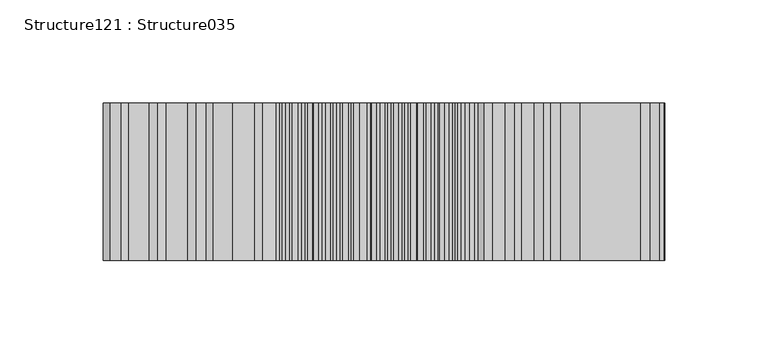
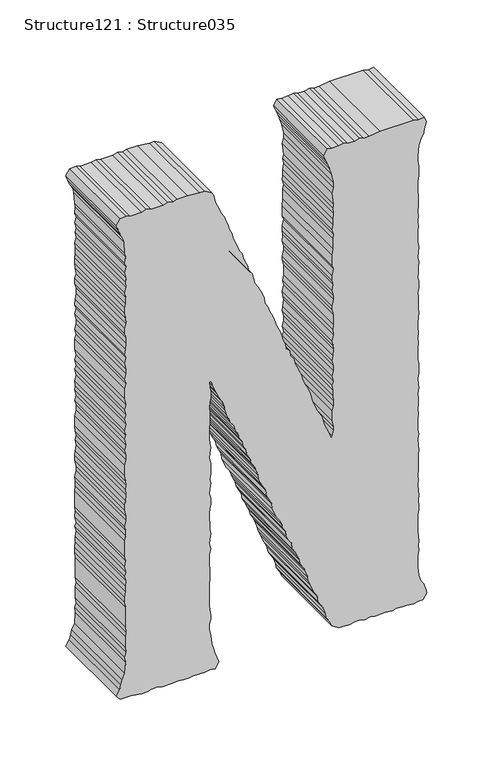
"""IFC4 building model written with IfcOpenShell, lengths in millimetres: proxy geometry, Structure121 : Structure035."""

from ifc_helpers import new_model, si_unit, frame, origin, place, context, project, spatial, polyline, outline, extrude, source, transform, mapped, element, save


def structure121_structure035_140282e5(model_context):
    return source(origin(), model_context, "Body", "SweptSolid", [
        extrude(outline(polyline([(3575.0851816, -43990.4752466), (3583.2863152, -43991.6353756), (3589.1527492, -43992.8163645), (3593.8285667, -43992.8163645), (3597.9540049, -43991.6353756), (3602.0280957, -43991.6353756), (3607.3393366, -43992.2371023), (3611.4134274, -43992.8163645), (3631.3410106, -43992.8163645), (3635.4407751, -43992.2371023), (3644.8245022, -43992.2371023), (3648.9258713, -43992.8163645), (3658.3015753, -43992.8163645), (3663.5598643, -43991.6353756), (3668.2437048, -43992.8163645), (3672.3691429, -43992.2371023), (3677.0449604, -43991.6353756), (3681.7271964, -43992.2371023), (3687.587212, -43992.2371023), (3691.6869765, -43992.8163645), (3696.3884676, -43992.8163645), (3700.4705815, -43992.2371023), (3704.5879966, -43991.6353756), (3709.8559132, -43991.6353756), (3714.5301261, -43992.8163645), (3718.6571688, -43992.2371023), (3723.9154578, -43991.6353756), (3728.0152223, -43992.2371023), (3732.7167134, -43991.6353756), (3742.6748889, -43991.6353756), (3747.3587295, -43992.8163645), (3752.6170184, -43992.2371023), (3757.3185096, -43991.6353756), (3760.818152, -43992.2371023), (3766.684586, -43992.8163645), (3774.8857196, -43992.8163645), (3780.7441306, -43992.2371023), (3790.1294623, -43992.2371023), (3794.2292268, -43992.8163645), (3798.9050443, -43992.2371023), (3803.0064134, -43991.6353756), (3808.8888934, -43991.6353756), (3812.9726119, -43992.2371023), (3818.2309008, -43992.8163645), (3817.6741031, -43991.6353756), (3812.9726119, -43989.2942576), (3808.290376, -43987.5340065), (3804.7730829, -43985.7962198), (3800.6717138, -43984.6152309), (3795.960595, -43981.6948508), (3790.7039107, -43979.9121352), (3787.2042683, -43978.7536107), (3782.5027771, -43977.5726218), (3777.8285642, -43975.8123707), (3773.7015215, -43974.0729794), (3770.2018791, -43971.1317394), (3766.1021146, -43969.9732149), (3760.2437036, -43967.632097), (3757.3185096, -43966.451108), (3752.6170184, -43964.1115947), (3748.5429276, -43962.9306058), (3743.8414364, -43960.5894878), (3739.1592005, -43960.0102256), (3733.8736333, -43957.09145), (3730.3563402, -43955.9104611), (3725.6741043, -43953.5484833), (3722.1568112, -43951.809092), (3716.8985223, -43950.0488409), (3712.7971532, -43949.4695787), (3708.087639, -43947.7093275), (3703.4134261, -43945.3682096), (3700.4705815, -43943.6079584), (3694.6298211, -43942.4269695), (3691.0868544, -43940.6667184), (3686.4030139, -43938.3256004), (3681.7271964, -43937.7463382), (3672.9435914, -43934.225836), (3668.8261762, -43931.2845959), (3664.1423357, -43929.5452046), (3660.6250426, -43928.3642157), (3655.9428067, -43926.0247024), (3651.8590883, -43925.4454402), (3647.1575971, -43923.1043222), (3643.6579547, -43920.7423444), (3638.3563415, -43920.1630822), (3634.2822506, -43917.8235688), (3630.1824862, -43916.0617131), (3625.472972, -43913.7221997), (3621.3732075, -43913.120473), (3616.69739, -43910.2016975), (3613.1720739, -43908.4398417), (3607.3393366, -43906.6795906), (3603.7963698, -43906.1003284), (3599.7126514, -43904.3400772), (3591.5131224, -43900.8179704), (3586.8116312, -43898.478457), (3581.5276686, -43897.2974681), (3577.4535778, -43894.9579547), (3573.3265351, -43892.6168368), (3568.0682461, -43890.8565857), (3563.9412034, -43890.2773234), (3559.2669905, -43887.3585479), (3555.1848766, -43885.5966921), (3551.0658569, -43879.7366765), (3551.0658569, -43875.6353074), (3550.4833855, -43870.3529494), (3551.6675836, -43865.6739227), (3551.6675836, -43862.1518158), (3550.4833855, -43856.8710624), (3551.6675836, -43852.1904311), (3550.4833855, -43848.089062), (3551.0658569, -43842.2290464), (3551.0658569, -43838.729404), (3550.4833855, -43832.8677838), (3551.6675836, -43829.3472815), (3551.0658569, -43824.0649235), (3551.0658569, -43819.965159), (3550.4833855, -43814.1260033), (3551.0658569, -43810.0021697), (3551.0658569, -43805.9024052), (3556.3417965, -43802.4027628), (3559.8671125, -43803.5612873), (3565.7094775, -43805.323143), (3569.2524442, -43807.6626564), (3575.0851816, -43809.4229075), (3583.2863152, -43810.6038964), (3593.2541183, -43810.6038964), (3598.5284533, -43809.4229075), (3602.0280957, -43810.0021697), (3607.3393366, -43809.4229075), (3611.4134274, -43810.0021697), (3616.69739, -43810.6038964), (3631.3410106, -43810.6038964), (3635.4407751, -43809.4229075), (3640.114988, -43809.4229075), (3644.2420307, -43810.0021697), (3650.1004418, -43809.4229075), (3653.6000842, -43810.0021697), (3659.4584952, -43810.6038964), (3662.9854159, -43810.0021697), (3668.2437048, -43810.6038964), (3672.3691429, -43810.0021697), (3687.0127636, -43810.0021697), (3691.0868544, -43809.4229075), (3695.786741, -43810.0021697), (3701.6547796, -43810.6038964), (3705.7545441, -43809.4229075), (3709.8559132, -43810.6038964), (3719.2316172, -43810.6038964), (3725.0996559, -43810.0021697), (3728.5992983, -43810.6038964), (3734.47536, -43810.0021697), (3739.1592005, -43810.0021697), (3743.8414364, -43810.6038964), (3748.5429276, -43809.4229075), (3752.04257, -43810.0021697), (3757.8753073, -43810.6038964), (3762.0023501, -43809.4229075), (3771.3860772, -43809.4229075), (3775.4874463, -43810.6038964), (3784.8438951, -43810.6038964), (3790.1294623, -43810.0021697), (3795.4037973, -43810.6038964), (3799.5051664, -43810.0021697), (3804.7730829, -43810.6038964), (3809.4729695, -43810.6038964), (3812.9726119, -43810.0021697), (3818.2309008, -43809.4229075), (3822.348316, -43810.0021697), (3832.3161191, -43810.0021697), (3836.9919366, -43810.6038964), (3841.0900965, -43809.4229075), (3846.9757858, -43809.4229075), (3850.4754282, -43810.6038964), (3855.7353217, -43810.0021697), (3859.8591552, -43810.0021697), (3865.1190488, -43809.4229075), (3869.8189354, -43810.6038964), (3879.1769888, -43809.4229075), (3883.8881076, -43810.6038964), (3893.246161, -43810.6038964), (3898.5301236, -43810.0021697), (3903.2059411, -43810.6038964), (3907.3313793, -43810.0021697), (3912.0071968, -43810.6038964), (3916.6653636, -43810.0021697), (3926.6492128, -43810.0021697), (3930.1745289, -43810.6038964), (3940.1166583, -43810.6038964), (3944.8165449, -43809.4229075), (3953.5937315, -43809.4229075), (3959.4617701, -43810.6038964), (3962.9774586, -43810.6038964), (3972.9372387, -43809.4229075), (3977.6194746, -43807.6626564), (3982.8793681, -43805.323143), (3986.4046842, -43804.7422762), (3992.2614906, -43802.9820251), (3996.9645864, -43804.7422762), (3996.390138, -43809.4229075), (3997.5486624, -43814.1260033), (3997.5486624, -43843.4100353), (3996.390138, -43852.7696933), (3996.390138, -43857.4727891), (3997.5486624, -43860.9932914), (3996.390138, -43865.6739227), (3996.390138, -43871.5339383), (3997.5486624, -43875.0335807), (3996.9645864, -43879.7366765), (3996.9645864, -43885.5966921), (3997.5486624, -43889.6980612), (3992.2614906, -43892.6168368), (3987.5792547, -43890.8565857), (3982.3225704, -43888.5170723), (3978.2035506, -43887.3585479), (3972.9372387, -43885.5966921), (3964.1343784, -43883.836441), (3959.4617701, -43883.836441), (3954.7506513, -43885.0174299), (3944.235678, -43883.836441), (3940.718385, -43884.4157032), (3936.0345445, -43883.836441), (3930.7329312, -43884.4157032), (3925.4746423, -43884.4157032), (3921.3748778, -43885.0174299), (3916.6653636, -43883.836441), (3912.5896682, -43884.4157032), (3903.2059411, -43884.4157032), (3897.3475301, -43885.0174299), (3887.9621984, -43885.0174299), (3884.4609514, -43883.836441), (3878.5784713, -43885.0174299), (3873.9203044, -43885.0174299), (3870.4030114, -43884.4157032), (3864.5446004, -43885.0174299), (3859.8591552, -43883.836441), (3856.3161885, -43883.836441), (3850.4754282, -43885.0174299), (3846.9757858, -43885.0174299), (3842.2758992, -43883.836441), (3832.8921721, -43883.836441), (3828.2163546, -43884.4157032), (3823.5341187, -43883.836441), (3818.2309008, -43885.0174299), (3813.5743386, -43884.4157032), (3810.0474179, -43883.836441), (3804.1890069, -43884.4157032), (3800.0876378, -43885.0174299), (3794.8309535, -43883.836441), (3790.1294623, -43883.836441), (3785.4456218, -43885.0174299), (3780.7441306, -43883.836441), (3777.2444882, -43885.0174299), (3772.5606477, -43884.4157032), (3767.2590344, -43884.4157032), (3762.5848215, -43883.836441), (3757.3185096, -43883.836441), (3753.8012165, -43885.0174299), (3744.4158848, -43885.0174299), (3738.5574738, -43883.836441), (3735.0578314, -43883.836441), (3730.3563402, -43885.0174299), (3729.1737467, -43886.1759543), (3733.2991849, -43887.9378101), (3739.1592005, -43890.2773234), (3743.2332913, -43892.0375746), (3752.04257, -43894.3786925), (3755.559863, -43896.7406703), (3760.2437036, -43899.0801837), (3764.9435901, -43900.8179704), (3768.4432325, -43902.5798261), (3773.11905, -43903.760815), (3777.8285642, -43904.9193395), (3781.9299333, -43906.6795906), (3786.0280932, -43909.0207085), (3791.8865042, -43911.3826864), (3795.4037973, -43911.9619486), (3799.5051664, -43913.7221997), (3803.5872802, -43915.4824508), (3808.290376, -43917.8235688), (3813.5743386, -43919.0045577), (3817.6741031, -43921.9233333), (3822.348316, -43922.5025955), (3825.2911606, -43925.4454402), (3830.5574726, -43926.6039646), (3834.6588416, -43928.3642157), (3838.7586061, -43929.5452046), (3844.0345457, -43931.2845959), (3848.7167816, -43933.6465737), (3851.6612309, -43934.8050982), (3857.5019912, -43936.5653493), (3860.4432313, -43937.7463382), (3864.5446004, -43940.0874562), (3869.8189354, -43941.8477073), (3874.5043805, -43944.1872207), (3879.1769888, -43944.7664829), (3883.2863809, -43946.5283386), (3890.905043, -43950.0488409), (3895.5888836, -43952.9676165), (3900.8648231, -43954.15021), (3904.9645876, -43955.3087344), (3909.0627475, -43958.2499745), (3914.3499193, -43959.4309634), (3917.8479571, -43961.1703547), (3922.5494483, -43962.9306058), (3926.6492128, -43964.1115947), (3930.1745289, -43966.451108), (3934.8503464, -43968.2113592), (3939.5325823, -43969.9732149), (3944.235678, -43972.3127283), (3947.7337158, -43972.8919905), (3952.9920048, -43975.2315038), (3957.1190475, -43976.4140974), (3961.2204166, -43978.1743485), (3966.5043792, -43979.9121352), (3971.1785921, -43982.8533752), (3974.7055128, -43984.0359687), (3978.8036727, -43985.7962198), (3982.8793681, -43987.5340065), (3988.7634528, -43988.7149954), (3992.2614906, -43990.4752466), (3995.7803883, -43996.916129), (3995.7803883, -44001.0174981), (3996.9645864, -44011.558145), (3996.9645864, -44020.9418721), (3995.7803883, -44024.4623744), (3996.9645864, -44029.1430057), (3995.7803883, -44033.2427702), (3995.7803883, -44043.7850217), (3996.9645864, -44047.8847862), (3995.7803883, -44051.9861553), (3995.7803883, -44061.9700045), (3996.9645864, -44065.4696469), (3996.390138, -44070.7504003), (3991.0788971, -44074.2500427), (3986.4046842, -44072.5106514), (3982.8793681, -44071.3296625), (3977.6194746, -44068.4108869), (3973.5197101, -44067.229898), (3962.9774586, -44066.6506358), (3959.4617701, -44066.0489091), (3953.5937315, -44066.6506358), (3950.0940891, -44065.4696469), (3944.8165449, -44066.6506358), (3940.1166583, -44065.4696469), (3936.0345445, -44066.0489091), (3931.3346579, -44065.4696469), (3926.6492128, -44066.6506358), (3921.9733953, -44066.0489091), (3916.0909152, -44066.0489091), (3912.5896682, -44066.6506358), (3907.3313793, -44066.6506358), (3902.6314927, -44066.0489091), (3897.3475301, -44065.4696469), (3893.822214, -44066.6506358), (3888.5623205, -44066.6506358), (3884.4609514, -44065.4696469), (3879.1769888, -44065.4696469), (3873.9203044, -44066.0489091), (3869.2444869, -44066.6506358), (3865.7015202, -44065.4696469), (3861.0192843, -44066.6506358), (3855.1769193, -44065.4696469), (3851.0595042, -44065.4696469), (3846.3772683, -44066.6506358), (3841.6741725, -44065.4696469), (3837.6000817, -44066.6506358), (3828.2163546, -44066.6506358), (3822.348316, -44065.4696469), (3818.2309008, -44066.6506358), (3812.9726119, -44065.4696469), (3809.4729695, -44066.6506358), (3804.1890069, -44065.4696469), (3798.9050443, -44066.6506358), (3794.2292268, -44066.0489091), (3790.7039107, -44066.6506358), (3784.8438951, -44065.4696469), (3780.7441306, -44066.6506358), (3776.0618947, -44065.4696469), (3771.3860772, -44065.4696469), (3766.684586, -44066.6506358), (3757.3185096, -44066.6506358), (3752.04257, -44066.0489091), (3747.9428055, -44065.4696469), (3743.8414364, -44066.0489091), (3739.1592005, -44065.4696469), (3733.8736333, -44066.0489091), (3729.7738688, -44066.6506358), (3725.0996559, -44066.6506358), (3719.2316172, -44065.4696469), (3715.7143242, -44065.4696469), (3709.8559132, -44066.6506358), (3706.3289925, -44066.0489091), (3701.6547796, -44066.0489091), (3696.9709391, -44066.6506358), (3682.3289231, -44066.6506358), (3678.2018803, -44066.0489091), (3672.9435914, -44066.6506358), (3667.6853024, -44065.4696469), (3664.1423357, -44066.6506358), (3659.4584952, -44065.4696469), (3654.7842823, -44066.0489091), (3649.5003197, -44066.0489091), (3644.8245022, -44066.6506358), (3640.114988, -44066.6506358), (3635.4407751, -44066.0489091), (3616.69739, -44066.0489091), (3612.0135494, -44065.4696469), (3607.8961343, -44066.0489091), (3597.9540049, -44066.0489091), (3593.2541183, -44065.4696469), (3589.1527492, -44066.6506358), (3584.4689087, -44066.0489091), (3574.5107332, -44066.6506358), (3569.2524442, -44068.9901491), (3565.1254015, -44070.1486736), (3561.025637, -44071.3296625), (3555.7416744, -44074.2500427), (3551.6675836, -44070.7504003), (3551.6675836, -44061.3682778), (3550.4833855, -44051.9861553), (3550.4833855, -44047.305524), (3551.6675836, -44043.7850217), (3551.6675836, -44037.9234015), (3550.4833855, -44033.8220324), (3550.4833855, -44025.0416366), (3551.0658569, -44019.7817431), (3550.4833855, -44015.6595141), (3550.4833855, -44010.3996206), (3551.0658569, -44006.8791183), (3551.0658569, -43996.916129), (3551.6675836, -43992.2371023), (3551.0658569, -43987.5340065), (3556.3417965, -43984.6152309), (3565.7094775, -43988.1357332), (3569.2524442, -43988.7149954), (3575.0851816, -43990.4752466)])), frame((0.0, 247945.1599557, 0.0), z_axis=(0.0, 1.0, 0.0), x_axis=(0.0, 0.0, 1.0)), (0.0, 0.0, 1.0), 76.2),
    ])


if __name__ == "__main__":
    model = new_model("IFC4")
    model_context = context("Model", 3, world=origin())
    ifc_project = project(units=[si_unit("LENGTHUNIT", "METRE", prefix="MILLI")], contexts=[model_context])
    site = spatial("IfcSite", under=ifc_project)
    building = spatial("IfcBuilding", under=site)
    placement = place(None, origin())
    structure121_structure035_shape = structure121_structure035_140282e5(model_context)
    element("IfcBuildingElementProxy", 1, Name="Structure121 : Structure035", ObjectType="Structure121 : Structure035", at=placement, inside=building, context=model_context, shape_type="MappedRepresentation", body=[
        mapped(structure121_structure035_shape, transform((0.0, 0.0, 0.0), x_axis=(1.0, 0.0, 0.0), y_axis=(0.0, 1.0, 0.0), z_axis=(0.0, 0.0, 1.0))),
    ])
    save(model, "model.ifc")

# Revit data of these elements
# Type "Structure121 : Structure035"
#   NameOverride = "Structure035"
# Element 1 (IfcBuildingElementProxy, "Structure121 : Structure035")
#   Materials on its faces: "BRUSHED ALUM. LETTERING"
# Materials
#   "BRUSHED ALUM. LETTERING": class "Unassigned", colour RGB 169 181 186, transparency 0, Cost = 0
